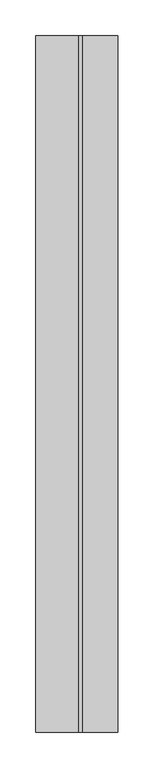
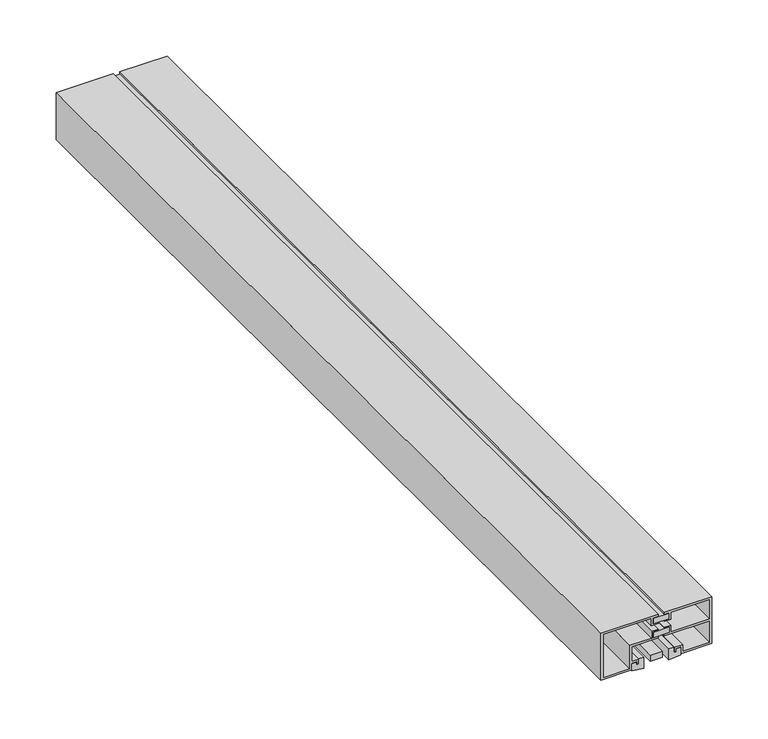
"""IFC4 building model written with IfcOpenShell, lengths in millimetres: proxy geometry, Generic Models 3:Generic Models 1:4:Generic Models 1:4 : Generic Models 3:Generic Models 1:300625:338780:Generic Models 1:4:Generic Models 1:4 : Generic Models 3:Generic Models 1:300625:338780 : Generic Models 3:Generic Models 1:4:Generic Models 1:4 : Generic Models 3:Generic Models 1:300625:338780:2 : Generic Models 3:Generic Models 1:4:Generic Models 1:4 : Generic Models 3:Generic Models 1:300625:338780:Generic Models 1:4:Generic Models 1:4 : Generic Models 3:Generic Models 1:300625:338780 : Generic Models 3:Generic Models 1:4:Generic Models 1:4 : Generic Models 3:Generic Models 1:300625:338780:301383."""

from ifc_helpers import new_model, si_unit, frame, origin, place, context, project, spatial, polyline, outline, extrude, source, transform, mapped, element, save


def generic_models_6ef09fd9(model_context):
    return source(origin(), model_context, "Body", "SweptSolid", [
        extrude(outline(polyline([(560318.3771075, -573566.7126607), (560302.2656713, -573566.7126607), (560302.2656713, -572596.7501607), (560318.3771075, -572596.7501607), (560318.3771075, -573566.7126607)])), frame((0.0, 0.0, 3693.6142952), z_axis=(0.0, 0.0, 1.0), x_axis=(1.0, 0.0, 0.0)), (0.0, 0.0, 1.0), 6.0797872),
        extrude(outline(polyline([(560318.4673755, -573566.7126607), (560302.3559394, -573566.7126607), (560302.3559394, -572596.7501607), (560318.4673755, -572596.7501607), (560318.4673755, -573566.7126607)])), frame((0.0, 0.0, 3678.5668218), z_axis=(0.0, 0.0, 1.0), x_axis=(1.0, 0.0, 0.0)), (0.0, 0.0, 1.0), 6.0797872),
        extrude(outline(polyline([(560311.6698356, -573566.7126607), (560298.9698356, -573566.7126607), (560298.9698356, -572596.7501607), (560311.6698356, -572596.7501607), (560311.6698356, -573566.7126607)])), frame((0.0, 0.0, 3654.1359064), z_axis=(0.0, 0.0, 1.0), x_axis=(1.0, 0.0, 0.0)), (0.0, 0.0, 1.0), 6.3435484),
        extrude(outline(polyline([(3650.2669395, 560280.3335989), (3648.8060727, 560292.2314048), (3660.8763298, 560292.2314048), (3660.8763298, 560287.4773489), (3655.1627892, 560287.4773489), (3655.1627892, 560284.6316707), (3658.1066489, 560284.6316707), (3658.1066489, 560280.3335989), (3650.2669395, 560280.3335989)])), frame((0.0, -573566.7126607, 0.0), z_axis=(0.0, 1.0, 0.0), x_axis=(0.0, 0.0, 1.0)), (0.0, 0.0, 1.0), 969.9625),
        extrude(outline(polyline([(3655.1627892, 560323.1623223), (3660.8763298, 560323.1623223), (3660.8763298, 560318.4082665), (3648.8060727, 560318.4082665), (3650.2669395, 560330.3060723), (3658.1066489, 560330.3060723), (3658.1066489, 560326.0080005), (3655.1627892, 560326.0080005), (3655.1627892, 560323.1623223)])), frame((0.0, -573566.7126607, 0.0), z_axis=(0.0, 1.0, 0.0), x_axis=(0.0, 0.0, 1.0)), (0.0, 0.0, 1.0), 969.9625),
        extrude(outline(polyline([(3651.2837766, 560362.4867239), (3702.05, 560362.4867239), (3702.05, 560313.5132777), (3699.6940824, 560313.5132777), (3699.6940824, 560318.3771075), (3693.6142952, 560318.3771075), (3693.6142952, 560313.5132777), (3692.3223404, 560313.5132777), (3692.3223404, 560320.277041), (3700.1277874, 560320.277041), (3700.1277874, 560360.5107931), (3678.5668218, 560360.5107931), (3678.5668218, 560320.367309), (3685.9385638, 560320.367309), (3685.9385638, 560313.6035457), (3684.646609, 560313.6035457), (3684.646609, 560318.4673755), (3678.5668218, 560318.4673755), (3678.5668218, 560313.6035457), (3676.6668883, 560313.6035457), (3676.6668883, 560360.5107931), (3653.1935757, 560360.5107931), (3653.1935757, 560332.6028808), (3660.4794548, 560332.6028808), (3660.4794548, 560323.5591973), (3655.5596642, 560323.5591973), (3655.5596642, 560325.6111255), (3658.5035239, 560325.6111255), (3658.5035239, 560330.7029473), (3651.2837766, 560330.7029473), (3651.2837766, 560362.4867239)])), frame((0.0, -573566.7126607, 0.0), z_axis=(0.0, 1.0, 0.0), x_axis=(0.0, 0.0, 1.0)), (0.0, 0.0, 1.0), 969.9625),
        extrude(outline(polyline([(3658.5035239, 560285.0285457), (3655.5596642, 560285.0285457), (3655.5596642, 560287.0804739), (3660.4794548, 560287.0804739), (3660.4794548, 560279.9367239), (3676.6668883, 560279.9367239), (3676.6668883, 560307.2197691), (3678.5668218, 560307.2197691), (3678.5668218, 560302.3559394), (3684.646609, 560302.3559394), (3684.646609, 560307.2197691), (3685.9385638, 560307.2197691), (3685.9385638, 560300.4560058), (3678.5668218, 560300.4560058), (3678.5668218, 560278.0367904), (3653.1837101, 560278.0367904), (3653.1837101, 560250.6946362), (3700.1500665, 560250.6946362), (3700.1500665, 560300.3657378), (3692.3223404, 560300.3657378), (3692.3223404, 560307.1295011), (3693.6142952, 560307.1295011), (3693.6142952, 560302.2656713), (3699.6940824, 560302.2656713), (3699.6940824, 560307.1295011), (3702.05, 560307.1295011), (3702.05, 560248.1867239), (3651.2837766, 560248.1867239), (3651.2837766, 560279.9367239), (3658.5035239, 560279.9367239), (3658.5035239, 560285.0285457)])), frame((0.0, -573566.7126607, 0.0), z_axis=(0.0, 1.0, 0.0), x_axis=(0.0, 0.0, 1.0)), (0.0, 0.0, 1.0), 969.9625),
    ])


if __name__ == "__main__":
    model = new_model("IFC4")
    model_context = context("Model", 3, world=origin())
    ifc_project = project(units=[si_unit("LENGTHUNIT", "METRE", prefix="MILLI")], contexts=[model_context])
    site = spatial("IfcSite", under=ifc_project)
    building = spatial("IfcBuilding", under=site)
    placement = place(None, origin())
    generic_models_shape = generic_models_6ef09fd9(model_context)
    element("IfcBuildingElementProxy", 1, Name="Generic Models 3:Generic Models 1:4:Generic Models 1:4 : Generic Models 3:Generic Models 1:300625:338780:Generic Models 1:4:Generic Models 1:4 : Generic Models 3:Generic Models 1:300625:338780 : Generic Models 3:Generic Models 1:4:Generic Models 1:4 : Generic Models 3:Generic Models 1:300625:338780:2 : Generic Models 3:Generic Models 1:4:Generic Models 1:4 : Generic Models 3:Generic Models 1:300625:338780:Generic Models 1:4:Generic Models 1:4 : Generic Models 3:Generic Models 1:300625:338780 : Generic Models 3:Generic Models 1:4:Generic Models 1:4 : Generic Models 3:Generic Models 1:300625:338780:301383", ObjectType="Generic Models 3:Generic Models 1:4:Generic Models 1:4 : Generic Models 3:Generic Models 1:300625:338780:Generic Models 1:4:Generic Models 1:4 : Generic Models 3:Generic Models 1:300625:338780 : Generic Models 3:Generic Models 1:4:Generic Models 1:4 : Generic Models 3:Generic Models 1:300625:338780:2 : Generic Models 3:Generic Models 1:4:Generic Models 1:4 : Generic Models 3:Generic Models 1:300625:338780:Generic Models 1:4:Generic Models 1:4 : Generic Models 3:Generic Models 1:300625:338780 : Generic Models 3:Generic Models 1:4:Generic Models 1:4 : Generic Models 3:Generic Models 1:300625:338780:301383", at=placement, inside=building, context=model_context, shape_type="MappedRepresentation", body=[
        mapped(generic_models_shape, transform((0.0, 0.0, 0.0), x_axis=(1.0, 0.0, 0.0), y_axis=(0.0, 1.0, 0.0), z_axis=(0.0, 0.0, 1.0))),
    ])
    save(model, "model.ifc")

# Revit data of these elements
# Type "Generic Models 3:Generic Models 1:4:Generic Models 1:4 : Generic Models 3:Generic Models 1:300625:338780:Generic Models 1:4:Generic Models 1:4 : Generic Models 3:Generic Models 1:300625:338780 : Generic Models 3:Generic Models 1:4:Generic Models 1:4 : Generic Models 3:Generic Models 1:300625:338780:2 : Generic Models 3:Generic Models 1:4:Generic Models 1:4 : Generic Models 3:Generic Models 1:300625:338780:Generic Models 1:4:Generic Models 1:4 : Generic Models 3:Generic Models 1:300625:338780 : Generic Models 3:Generic Models 1:4:Generic Models 1:4 : Generic Models 3:Generic Models 1:300625:338780:301383"
#   NameOverride = "Generic Models 3:Generic Models 1:4:Generic Models 1:4 : Generic Models 3:Generic Models 1:300625:338780:Generic Models 1:4:Generic Models 1:4 : Generic Models 3:Generic Models 1:300625:338780 : Generic Models 3:Generic Models 1:4:Generic Models 1:4 : Generic Models 3:Generic Models 1:300625:338780:301383"
#   ObjectTypeOverride = "Generic Models 1:4:Generic Models 1:4 : Generic Models 3:Generic Models 1:300625:338780 : Generic Models 3:Generic Models 1:4:Generic Models 1:4 : Generic Models 3:Generic Models 1:300625:338780"
#   Reference = "Generic Models 1"
#   Tag = "301383"
# Element 1 (IfcBuildingElementProxy, "Generic Models 3:Generic Models 1:4:Generic Models 1:4 : Generic Models 3:Generic Models 1:300625:338780:Generic Models 1:4:Generic Models 1:4 : Generic Models 3:Generic Models 1:300625:338780 : Generic Models 3:Generic Models 1:4:Generic Models 1:4 : Generic Models 3:Generic Models 1:300625:338780:2 : Generic Models 3:Generic Models 1:4:Generic Models 1:4 : Generic Models 3:Generic Models 1:300625:338780:Generic Models 1:4:Generic Models 1:4 : Generic Models 3:Generic Models 1:300625:338780 : Generic Models 3:Generic Models 1:4:Generic Models 1:4 : Generic Models 3:Generic Models 1:300625:338780:301383")
#   Materials on its faces: "THERMAL BROKEN ALUMINUM STOREFRONT"
# Materials
#   "THERMAL BROKEN ALUMINUM STOREFRONT": class "Unassigned", colour RGB 244 244 244, transparency 0, Cost = 0
